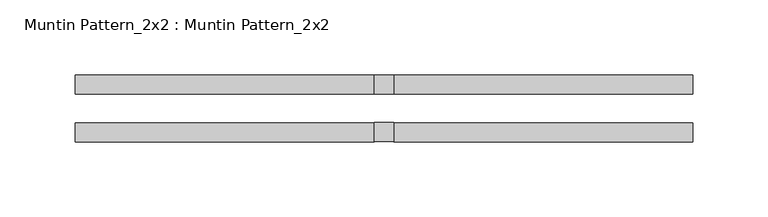
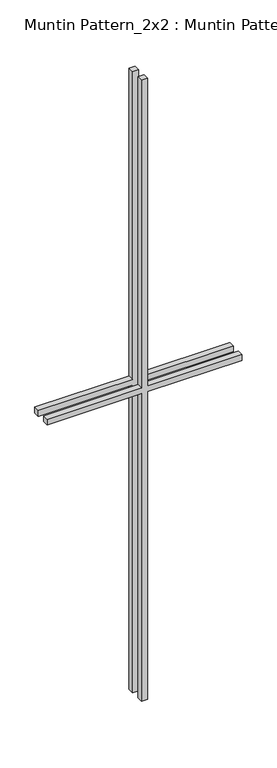
"""IFC4 building model written with IfcOpenShell, lengths in millimetres: proxy geometry, Muntin Pattern_2x2 : Muntin Pattern_2x2."""

import ifcopenshell
import ifcopenshell.guid

model = None  # the IFC model being written
_history = None  # IfcOwnerHistory: only IFC2X3 demands one
_inside = {}  # id of a spatial element -> (the spatial element, [elements in it])
_under = {}  # id of a project, library or spatial element -> (it, [spatial elements below it])
_declared = {}  # id of a project -> (the project, [libraries it declares])
_typed = {}  # id of a type object -> (the type object, [elements of that type])
_made_of = {}  # id of a material, layer set ... -> (it, [elements and type objects made of it])


def new_model(schema):
    """Start an empty IFC model of exactly this schema.

    Asked for "IFC4X3", IfcOpenShell would pick the latest addendum, in which some entities
    have other attributes; the version numbers below select the first issue.
    IFC2X3 requires an IfcOwnerHistory on every rooted entity: one is made here for all.
    """
    global model, _history
    if schema == "IFC4X3":
        model = ifcopenshell.file(schema_version=(4, 3, 0, 0))
    else:
        model = ifcopenshell.file(schema=schema)
    _inside.clear()
    _under.clear()
    _declared.clear()
    _typed.clear()
    _made_of.clear()
    _history = None
    if model.schema == "IFC2X3":
        org = make("IfcOrganization", Name="unknown")
        user = make(
            "IfcPersonAndOrganization",
            ThePerson=make("IfcPerson", FamilyName="unknown"),
            TheOrganization=org,
        )
        app = make(
            "IfcApplication",
            ApplicationDeveloper=org,
            Version="unknown",
            ApplicationFullName="unknown",
            ApplicationIdentifier="unknown",
        )
        _history = make(
            "IfcOwnerHistory",
            OwningUser=user,
            OwningApplication=app,
            ChangeAction="ADDED",
            CreationDate=0,
        )
    return model


def make(cls, **values):
    """One entity of the class cls with the attributes given. An attribute that is None is left unset."""
    return model.create_entity(
        cls, **{name: value for name, value in values.items() if value is not None}
    )


def rooted(cls, **values):
    """An entity with a GlobalId (a new one), such as an element, a storey or a relation."""
    return make(cls, GlobalId=ifcopenshell.guid.new(), OwnerHistory=_history, **values)


def si_unit(unit_type, name, prefix=None):
    """IfcSIUnit, for example si_unit("LENGTHUNIT", "METRE", prefix="MILLI")."""
    return make("IfcSIUnit", UnitType=unit_type, Prefix=prefix, Name=name)


def assignment(units):
    """IfcUnitAssignment: the units of a project."""
    return None if units is None else make("IfcUnitAssignment", Units=units)


def point(xyz):
    """IfcCartesianPoint."""
    return None if xyz is None else make("IfcCartesianPoint", Coordinates=xyz)


def direction(xyz):
    """IfcDirection."""
    return None if xyz is None else make("IfcDirection", DirectionRatios=xyz)


def frame(location, z_axis=None, x_axis=None):
    """IfcAxis2Placement3D, a coordinate frame: its origin and axes. An axis left out is left unset."""
    return make(
        "IfcAxis2Placement3D",
        Location=point(location),
        Axis=direction(z_axis),
        RefDirection=direction(x_axis),
    )


def origin():
    """The frame at (0, 0, 0) with its axes left unset."""
    return frame((0.0, 0.0, 0.0))


def place(relative_to, where):
    """IfcLocalPlacement: puts the frame where relative to a parent placement (None: the world)."""
    return make(
        "IfcLocalPlacement", PlacementRelTo=relative_to, RelativePlacement=where
    )


def context(
    kind, dimensions, precision=None, world=None, true_north=None, identifier=None
):
    """IfcGeometricRepresentationContext, for example the 3D "Model" context."""
    return make(
        "IfcGeometricRepresentationContext",
        ContextIdentifier=identifier,
        ContextType=kind,
        CoordinateSpaceDimension=dimensions,
        Precision=precision,
        WorldCoordinateSystem=world,
        TrueNorth=true_north,
    )


def project(units=None, contexts=None):
    """IfcProject with its units and contexts."""
    return rooted(
        "IfcProject",
        Name="project",
        RepresentationContexts=contexts,
        UnitsInContext=assignment(units),
    )


def spatial(cls, under=None, at=None, **own):
    """A site, building, storey or space (cls), placed at a placement, below another one or the project."""
    s = rooted(cls, ObjectPlacement=at, **own)
    if under is not None:
        _under.setdefault(under.id(), (under, []))[1].append(s)
    return s


def polyline(points):
    """IfcPolyline through the points."""
    return make("IfcPolyline", Points=[point(p) for p in points])


def outline(outer, holes=None, kind="AREA"):
    """IfcArbitraryClosedProfileDef: a profile drawn as a closed curve; with holes, ...WithVoids."""
    if holes is None:
        return make("IfcArbitraryClosedProfileDef", ProfileType=kind, OuterCurve=outer)
    return make(
        "IfcArbitraryProfileDefWithVoids",
        ProfileType=kind,
        OuterCurve=outer,
        InnerCurves=holes,
    )


def extrude(swept, where, along, depth):
    """IfcExtrudedAreaSolid: the profile swept, set in the frame where, extruded along a direction by depth."""
    return make(
        "IfcExtrudedAreaSolid",
        SweptArea=swept,
        Position=where,
        ExtrudedDirection=direction(along),
        Depth=depth,
    )


def shape(context_of_items, identifier, shape_type, items):
    """IfcShapeRepresentation: the items that make up one representation, for example the "Body"."""
    return make(
        "IfcShapeRepresentation",
        ContextOfItems=context_of_items,
        RepresentationIdentifier=identifier,
        RepresentationType=shape_type,
        Items=items,
    )


def source(mapping_origin, context_of_items, identifier, shape_type, items):
    """IfcRepresentationMap: a shape defined once, which mapped items show again and again."""
    return make(
        "IfcRepresentationMap",
        MappingOrigin=mapping_origin,
        MappedRepresentation=shape(context_of_items, identifier, shape_type, items),
    )


def transform(
    local_origin,
    x_axis=None,
    y_axis=None,
    z_axis=None,
    scale=None,
    scale2=None,
    scale3=None,
    uniform=True,
):
    """IfcCartesianTransformationOperator3D, or its non-uniform kind. x_axis, y_axis, z_axis: its Axis1, 2, 3."""
    if uniform:
        return make(
            "IfcCartesianTransformationOperator3D",
            Axis1=direction(x_axis),
            Axis2=direction(y_axis),
            LocalOrigin=point(local_origin),
            Scale=scale,
            Axis3=direction(z_axis),
        )
    return make(
        "IfcCartesianTransformationOperator3DnonUniform",
        Axis1=direction(x_axis),
        Axis2=direction(y_axis),
        LocalOrigin=point(local_origin),
        Scale=scale,
        Axis3=direction(z_axis),
        Scale2=scale2,
        Scale3=scale3,
    )


def mapped(mapping_source, mapping_target):
    """IfcMappedItem: shows the shape of a source again, moved by a transform."""
    return make(
        "IfcMappedItem", MappingSource=mapping_source, MappingTarget=mapping_target
    )


def made_of(thing, what):
    """Note that an element or type object is made of a material, layer set ...; save() writes the relation."""
    if what is not None:
        _made_of.setdefault(what.id(), (what, []))[1].append(thing)
    return thing


def element(
    cls,
    number,
    at=None,
    inside=None,
    cuts=None,
    type_object=None,
    material=None,
    context=None,
    identifier="Body",
    shape_type=None,
    held_by="IfcProductDefinitionShape",
    body=None,
    shapes=None,
    **own,
):
    """One element of the class cls, such as IfcWall. Its Tag is "e" and its number.

    at: its placement. inside: the storey or other place that contains it. cuts: it is an
    opening in that element (IfcRelVoidsElement). A single representation is given by context,
    identifier, shape_type and body (its items); several are given by shapes. held_by: the class
    of the entity that holds the representations. save() writes the other relations.
    """
    e = rooted(cls, Tag="e%d" % number, ObjectPlacement=at, **own)
    if body is not None:
        shapes = [shape(context, identifier, shape_type, body)]
    if shapes is not None:
        e.Representation = make(held_by, Representations=shapes)
    if inside is not None:
        _inside.setdefault(inside.id(), (inside, []))[1].append(e)
    if cuts is not None:
        rooted(
            "IfcRelVoidsElement", RelatingBuildingElement=cuts, RelatedOpeningElement=e
        )
    if type_object is not None:
        _typed.setdefault(type_object.id(), (type_object, []))[1].append(e)
    return made_of(e, material)


def aggregate(whole, parts):
    """IfcRelAggregates: a whole, such as a stair, and the parts it consists of."""
    return rooted("IfcRelAggregates", RelatingObject=whole, RelatedObjects=parts)


def save(model, path):
    """Write the relations noted so far, then the file.

    IfcRelAggregates (storeys below a building ...), IfcRelContainedInSpatialStructure (elements
    in a storey), IfcRelDefinesByType, IfcRelAssociatesMaterial and IfcRelDeclares: one each for
    every whole, place, type object, material and project.
    """
    for whole, parts in _under.values():
        aggregate(whole, parts)
    for where, things in _inside.values():
        rooted(
            "IfcRelContainedInSpatialStructure",
            RelatedElements=things,
            RelatingStructure=where,
        )
    for kind, things in _typed.values():
        rooted("IfcRelDefinesByType", RelatedObjects=things, RelatingType=kind)
    for what, things in _made_of.values():
        rooted("IfcRelAssociatesMaterial", RelatedObjects=things, RelatingMaterial=what)
    for by, libraries in _declared.values():
        rooted("IfcRelDeclares", RelatingContext=by, RelatedDefinitions=libraries)
    model.write(path)


def muntin_pattern_2x2_muntin_pattern_2x2_63bd3b25(model_context):
    return source(origin(), model_context, "Body", "SweptSolid", [
        extrude(outline(polyline([(698.5, -6.35), (698.5, -205.5885801), (685.8, -205.5885801), (685.8, -6.35), (0.0, -6.35), (0.0, 6.35), (685.8, 6.35), (685.8, 205.5885801), (698.5, 205.5885801), (698.5, 6.35), (1384.3, 6.35), (1384.3, -6.35), (698.5, -6.35)])), frame((0.0, 9.525, 0.0), z_axis=(0.0, 1.0, 0.0), x_axis=(0.0, 0.0, 1.0)), (0.0, 0.0, 1.0), 12.7),
        extrude(outline(polyline([(698.5, -6.35), (698.5, -205.5885801), (685.8, -205.5885801), (685.8, -6.35), (0.0, -6.35), (0.0, 6.35), (685.8, 6.35), (685.8, 205.5885801), (698.5, 205.5885801), (698.5, 6.35), (1384.3, 6.35), (1384.3, -6.35), (698.5, -6.35)])), frame((0.0, -22.225, 0.0), z_axis=(0.0, 1.0, 0.0), x_axis=(0.0, 0.0, 1.0)), (0.0, 0.0, 1.0), 12.7),
    ])


if __name__ == "__main__":
    model = new_model("IFC4")
    model_context = context("Model", 3, world=origin())
    ifc_project = project(units=[si_unit("LENGTHUNIT", "METRE", prefix="MILLI")], contexts=[model_context])
    site = spatial("IfcSite", under=ifc_project)
    building = spatial("IfcBuilding", under=site)
    placement = place(None, origin())
    muntin_pattern_2x2_muntin_pattern_2x2_shape = muntin_pattern_2x2_muntin_pattern_2x2_63bd3b25(model_context)
    element("IfcBuildingElementProxy", 1, Name="Muntin Pattern_2x2 : Muntin Pattern_2x2", ObjectType="Muntin Pattern_2x2 : Muntin Pattern_2x2", at=placement, inside=building, context=model_context, shape_type="MappedRepresentation", body=[
        mapped(muntin_pattern_2x2_muntin_pattern_2x2_shape, transform((0.0, 0.0, 0.0), x_axis=(1.0, 0.0, 0.0), y_axis=(0.0, 1.0, 0.0), z_axis=(0.0, 0.0, 1.0))),
    ])
    save(model, "model.ifc")

# Revit data of these elements
# Type "Muntin Pattern_2x2 : Muntin Pattern_2x2"
#   Width [instance default] = 4' - 0"
#   Thickness = 0' - 0 1/2"
#   Height [instance default] = 4' - 0"
#   Distance = 0' - 0 3/4"
#   Interior Material [instance default] = none
#   Exterior Material [instance default] = none
#   Default Elevation = 0
# Element 1 (IfcBuildingElementProxy, "Muntin Pattern_2x2 : Muntin Pattern_2x2")
#   Width = 1' - 4.18808"
#   Height = 4' - 6 1/2"
#   Interior Material = Wood - Stained
#   Exterior Material = Clad - White
#   Materials on its faces: "Clad - White", "Wood - Stained"
# Materials
#   "Clad - White": class "Wood", colour RGB 242 242 238, transparency 0, Cost = 0
#   "Wood - Stained": class "Wood", colour RGB 224 178 126, transparency 0, Cost = 0
